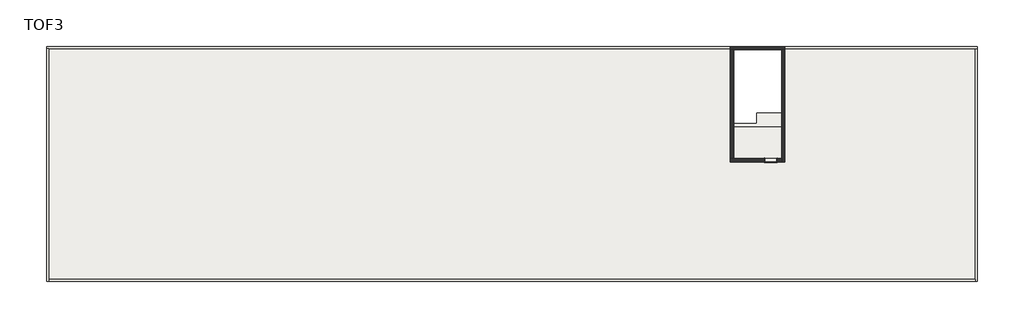
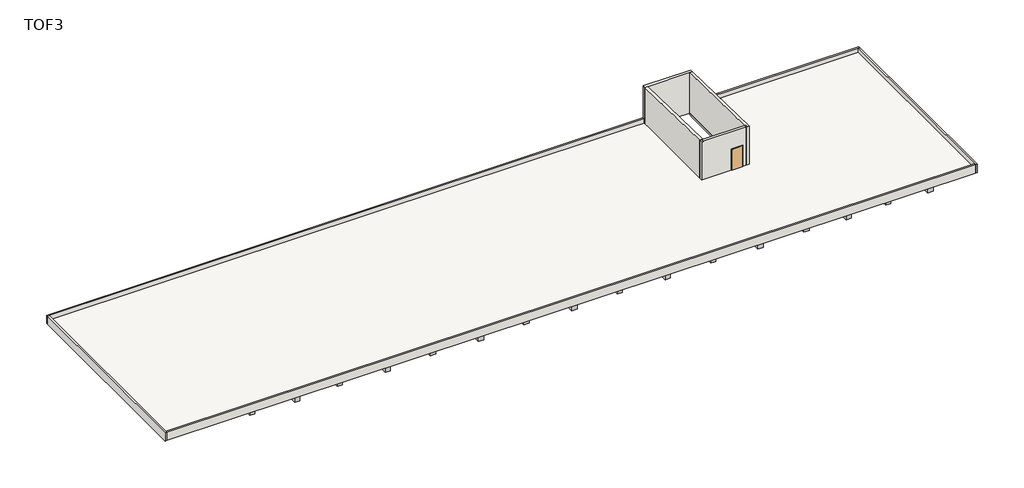
# One storey: 29 beams, 9 walls, 4 slabs, 1 door.
# Revit data of these elements (continued)
# Type "H_WA_AR_B02_Ext Wall_RC T150_parapet" (continued)
#   H_WM Code_3 = "A03AD035-00001 |  | M2 | Concrete Work | Substructure Work | Form Work (3 times in use) | Flat Form | Dressed Lumber, Plywood or Steel Form(Wood Planks are not Allowed) incl. Chamfer |  |  |  | A03AD035-00001 Concrete Work Substructure Work Form Work (3 times in use) Flat Form     Dressed Lumber, Plywood or Steel Form(Wood Planks are not Allowed) incl. Chamfer   |"
#   H_WM Code_4 = "A03AH056-00001 |  | M2 | Concrete Work | Concrete Protective Coating (U/G) | Bitumen/Bituminous/Asphalt Coating |  |  | A03AH056-00001 Concrete Work Concrete Protective Coating (U/G) Bitumen/Bituminous/Asphalt Coating         |"
#   H_WM Code_5 = "A01ZZ003-00001 |  | M3 | Earth Work | - | Backfill | Re-use, Soil |  |  |  | Compaction=(  )% |  | A01ZZ003-00001 Earth Work - Backfill Re-use, Soil        | Compaction=( 95 )%"
#   H_WM Code_6 = "A01ZZ004-00001 |  | M3 | Earth Work | - | Disposal | Soil |  |  |  | Disposal Distance=Appx. (  )km from Site |  | A01ZZ004-00001 Earth Work - Disposal Soil        | Disposal Distance=Appx. (20 )km from Site"
#   H_Rebar ratio = 0.12
#   Layers, outside or top first: 150 mm "00_Concrete_Reinf. Conc." (function 1)
# Elements 1, 2, 3, 4, 6, 7, 8, 9, 10, 11, 12, 13, 14 (IfcBeam, "RC Beam_Rectangular : H_SB_AR_S16_AG_B450xH700_RG1")
#   Comments = ""
#   hec_material3 = none
#   hec_material2 = none
#   hec_material1 = none
#   Structural Material = none
#   Phase Created = New Construction
# Element 5 (IfcBeam, "RC Beam_Rectangular : H_SB_AR_S16_AG_B450xH700_RB2")
#   Comments = ""
#   hec_material3 = none
#   hec_material2 = none
#   hec_material1 = none
#   Structural Material = none
#   Phase Created = New Construction
# Elements 15, 17, 19, 21, 23, 28, 29 (IfcBeam, "RC Beam_Rectangular : H_SB_AR_S16_AG_B450xH700_RB1")
#   Comments = ""
#   hec_material3 = none
#   hec_material2 = none
#   hec_material1 = none
#   Structural Material = none
#   Phase Created = New Construction
# Elements 16, 18, 20, 22, 24, 25, 26, 27 (IfcBeam, "RC Beam_Rectangular : H_SB_AR_S16_AG_B450xH700_RB1A")
#   Comments = ""
#   hec_material3 = none
#   hec_material2 = none
#   hec_material1 = none
#   Structural Material = none
#   Phase Created = New Construction
# Element 30 (IfcDoor, "Single Door_Steel : H_DR_AR_B12_Single Door_Steel_W1000xH2280_FSD2")
#   Phase Created = New Construction
# Element 31 (IfcSlab, "H_FL_AR_S17_RC Slab T150_RS1")
#   Comments = ""
#   TMP_Element Name = "SS2"
#   Height Offset From Level = 0 mm
#   built-in parameter 1001954 = 1
#   Phase Created = New Construction
#   Materials on its faces: "00_Concrete_Reinf. Conc."
# Element 32 (IfcSlab, "H_FL_AR_S17_RC Slab T200_SS1")
#   Comments = ""
#   TMP_Element Name = "SS2"
#   built-in parameter 1001955 = 3.14159 (stored number, unit not read)
#   Height Offset From Level = -4000 mm
#   built-in parameter 1001954 = 1
#   Phase Created = New Construction
#   Materials on its faces: "00_Concrete_Reinf. Conc."
# Element 33 (IfcSlab, "H_FL_AR_S17_RC Slab T200_SS1")
#   Comments = ""
#   TMP_Element Name = "SS2"
#   built-in parameter 1001955 = 3.14159 (stored number, unit not read)
#   Height Offset From Level = 0 mm
#   built-in parameter 1001954 = 1
#   Phase Created = New Construction
#   Materials on its faces: "00_Concrete_Reinf. Conc."
# Element 34 (IfcSlab, "H_RF_AR_B06_Roof Finish")
#   Height Offset From Level = 350 mm
#   Phase Created = New Construction
#   Materials on its faces: "Roofs"
# Element 35 (IfcWall, "H_WA_AR_B02_Ext Wall_RC T250_W1_PH")
#   Top Offset = -160 mm
#   Base Offset = 0 mm
#   wall height = 3640 mm
#   Phase Created = New Construction
#   Base Constraint = TOF3
#   Top Constraint = TOF4
#   Materials on its faces: "00_Concrete_Reinf. Conc."
# Elements 36, 37, 38 (IfcWall, "H_WA_AR_B02_Ext Wall_RC T250_W1_PH")
#   Top Offset = 0 mm
#   Base Offset = 0 mm
#   wall height = 3800 mm
#   Phase Created = New Construction
#   Base Constraint = TOF3
#   Top Constraint = TOF4
#   Materials on its faces: "00_Concrete_Reinf. Conc."
# Elements 39, 40, 41, 42, 43 (IfcWall, "H_WA_AR_B02_Ext Wall_RC T150_parapet")
#   Comments = ""
#   Top Offset = 150 mm
#   Base Offset = 0 mm
#   Unconnected Height = 740 mm
#   wall height = 740 mm
#   Phase Created = New Construction
#   Base Constraint = TOF3
#   Materials on its faces: "00_Concrete_Reinf. Conc."
# Materials
#   "00_Concrete_Reinf. Conc.": class "Concrete", colour RGB 176 176 176, transparency 0, Description = "Reinf. Conc.", Cost = 0, Image = Concrete.Cast-In-Place.Flat.Polished.Grey.jpg
#   "Roofs": class "Unassigned", colour RGB 38 15 153, transparency 0.5
